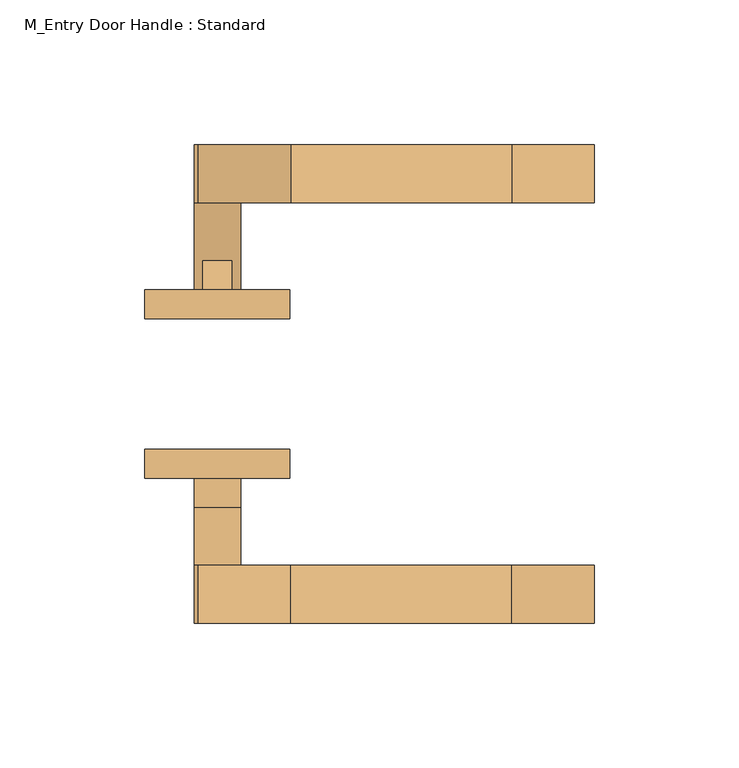
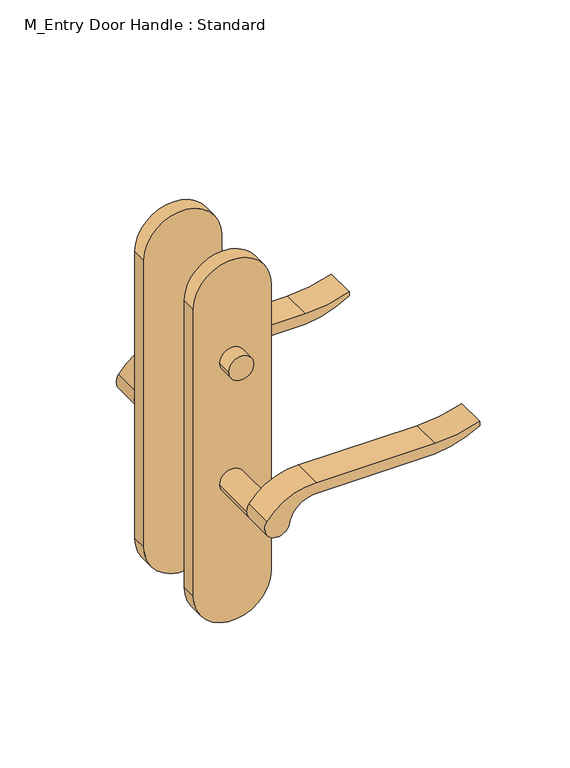
"""IFC4 building model written with IfcOpenShell, lengths in millimetres: door geometry, M_Entry Door Handle : Standard."""

from ifc_helpers import new_model, si_unit, point, frame, frame_2d, origin, origin_2d, place, context, project, spatial, polyline, circle_curve, trimmed, segment, composite_curve, outline, extrude, source, transform, mapped, element, save


def m_entry_door_handle_standard_7ac350b3(model_context):
    return source(origin(), model_context, "Body", "SweptSolid", [
        extrude(outline(polyline([(-5.0, 42.5), (5.0, 42.5), (5.0, 32.5), (-5.0, 32.5), (-5.0, 42.5)])), frame((0.0, 0.0, 67.5), z_axis=(0.0, 0.0, 1.0), x_axis=(1.0, 0.0, 0.0)), (0.0, 0.0, 1.0), 30.0),
        extrude(outline(composite_curve([segment(trimmed(circle_curve(frame_2d((82.5, 0.0)), 8.0), [point((82.5, 8.0))], [point((82.5, -8.0))], False, "CARTESIAN"), True, "CONTINUOUS"), segment(trimmed(circle_curve(frame_2d((82.5, 0.0)), 8.0), [point((82.5, -8.0))], [point((82.5, 8.0))], False, "CARTESIAN"), True, "CONTINUOUS")], self_intersect=False)), frame((0.0, -42.5, 0.0), z_axis=(0.0, 1.0, 0.0), x_axis=(0.0, 0.0, 1.0)), (0.0, 0.0, 1.0), 10.0),
        extrude(outline(composite_curve([segment(trimmed(circle_curve(origin_2d(), 8.0), [point((4.6523287, -6.5081363))], [point((0.0, 8.0))], False, "CARTESIAN"), True, "CONTINUOUS"), segment(trimmed(circle_curve(frame_2d((-5.1261387, 25.3861901)), 18.1261387), [point((0.0, 8.0))], [point((13.0, 25.3861901))], True, "CARTESIAN"), True, "CONTINUOUS"), segment(polyline([(13.0, 25.3861901), (13.0, 101.6435909)]), True, "CONTINUOUS"), segment(trimmed(circle_curve(frame_2d((72.2709207, 98.0603388)), 59.3791355), [point((13.0, 101.6435909))], [point((22.2135558, 130.0))], False, "CARTESIAN"), True, "CONTINUOUS"), segment(polyline([(22.2135558, 130.0), (25.0, 130.0)]), True, "CONTINUOUS"), segment(trimmed(circle_curve(frame_2d((103.2850638, 101.5772091)), 83.2850902), [point((25.0, 130.0))], [point((20.0, 101.6435909))], True, "CARTESIAN"), True, "CONTINUOUS"), segment(polyline([(20.0, 101.6435909), (20.0, 25.3674333)]), True, "CONTINUOUS"), segment(trimmed(circle_curve(frame_2d((-17.2444479, 23.6675129)), 37.2832219), [point((20.0, 25.3674333))], [point((4.6523287, -6.5081363))], False, "CARTESIAN"), True, "CONTINUOUS")], self_intersect=False)), frame((0.0, 62.5, 0.0), z_axis=(0.0, 1.0, 0.0), x_axis=(0.0, 0.0, 1.0)), (0.0, 0.0, 1.0), 20.0),
        extrude(outline(composite_curve([segment(trimmed(circle_curve(frame_2d((-5.1261318, 25.3861878)), 18.1261318), [point((-9.7e-06, 8.0))], [point((13.0, 25.3861878))], True, "CARTESIAN"), True, "CONTINUOUS"), segment(polyline([(13.0, 25.3861878), (13.0, 101.6435909)]), True, "CONTINUOUS"), segment(trimmed(circle_curve(frame_2d((72.2709207, 98.0603388)), 59.3791355), [point((13.0, 101.6435909))], [point((22.2135558, 130.0))], False, "CARTESIAN"), True, "CONTINUOUS"), segment(polyline([(22.2135558, 130.0), (25.0, 130.0)]), True, "CONTINUOUS"), segment(trimmed(circle_curve(frame_2d((103.2850638, 101.5772091)), 83.2850902), [point((25.0, 130.0))], [point((20.0, 101.6435909))], True, "CARTESIAN"), True, "CONTINUOUS"), segment(polyline([(20.0, 101.6435909), (20.0, 25.3674333)]), True, "CONTINUOUS"), segment(trimmed(circle_curve(frame_2d((-17.2444479, 23.6675129)), 37.2832219), [point((20.0, 25.3674333))], [point((4.6523287, -6.5081363))], False, "CARTESIAN"), True, "CONTINUOUS"), segment(trimmed(circle_curve(origin_2d(), 8.0), [point((4.6523287, -6.5081363))], [point((-9.7e-06, 8.0))], False, "CARTESIAN"), True, "CONTINUOUS")], self_intersect=False)), frame((0.0, -82.5, 0.0), z_axis=(0.0, 1.0, 0.0), x_axis=(0.0, 0.0, 1.0)), (0.0, 0.0, 1.0), 20.0),
        extrude(outline(composite_curve([segment(trimmed(circle_curve(origin_2d(), 8.0), [point((0.0, 8.0))], [point((0.0, -8.0))], False, "CARTESIAN"), True, "CONTINUOUS"), segment(trimmed(circle_curve(origin_2d(), 8.0), [point((0.0, -8.0))], [point((0.0, 8.0))], False, "CARTESIAN"), True, "CONTINUOUS")], self_intersect=False)), frame((0.0, 32.5, 0.0), z_axis=(0.0, 1.0, 0.0), x_axis=(0.0, 0.0, 1.0)), (0.0, 0.0, 1.0), 30.0),
        extrude(outline(composite_curve([segment(trimmed(circle_curve(origin_2d(), 8.0), [point((0.0, 8.0))], [point((0.0, -8.0))], False, "CARTESIAN"), True, "CONTINUOUS"), segment(trimmed(circle_curve(origin_2d(), 8.0), [point((0.0, -8.0))], [point((0.0, 8.0))], False, "CARTESIAN"), True, "CONTINUOUS")], self_intersect=False)), frame((0.0, -62.5, 0.0), z_axis=(0.0, 1.0, 0.0), x_axis=(0.0, 0.0, 1.0)), (0.0, 0.0, 1.0), 30.0),
        extrude(outline(composite_curve([segment(trimmed(circle_curve(frame_2d((-70.0, 0.0)), 25.0), [point((-70.0, -25.0))], [point((-70.0, 25.0))], False, "CARTESIAN"), True, "CONTINUOUS"), segment(polyline([(-70.0, 25.0), (125.0, 25.0)]), True, "CONTINUOUS"), segment(trimmed(circle_curve(frame_2d((125.0, 0.0)), 25.0), [point((125.0, 25.0))], [point((125.0, -25.0))], False, "CARTESIAN"), True, "CONTINUOUS"), segment(polyline([(125.0, -25.0), (-70.0, -25.0)]), True, "CONTINUOUS")], self_intersect=False)), frame((0.0, 22.5, 0.0), z_axis=(0.0, 1.0, 0.0), x_axis=(0.0, 0.0, 1.0)), (0.0, 0.0, 1.0), 10.0),
        extrude(outline(composite_curve([segment(trimmed(circle_curve(frame_2d((-70.0, 0.0)), 25.0), [point((-70.0, -25.0))], [point((-70.0, 25.0))], False, "CARTESIAN"), True, "CONTINUOUS"), segment(polyline([(-70.0, 25.0), (125.0, 25.0)]), True, "CONTINUOUS"), segment(trimmed(circle_curve(frame_2d((125.0, 0.0)), 25.0), [point((125.0, 25.0))], [point((125.0, -25.0))], False, "CARTESIAN"), True, "CONTINUOUS"), segment(polyline([(125.0, -25.0), (-70.0, -25.0)]), True, "CONTINUOUS")], self_intersect=False)), frame((0.0, -32.5, 0.0), z_axis=(0.0, 1.0, 0.0), x_axis=(0.0, 0.0, 1.0)), (0.0, 0.0, 1.0), 10.0),
    ])


if __name__ == "__main__":
    model = new_model("IFC4")
    model_context = context("Model", 3, world=origin())
    ifc_project = project(units=[si_unit("LENGTHUNIT", "METRE", prefix="MILLI")], contexts=[model_context])
    site = spatial("IfcSite", under=ifc_project)
    building = spatial("IfcBuilding", under=site)
    placement = place(None, origin())
    m_entry_door_handle_standard_shape = m_entry_door_handle_standard_7ac350b3(model_context)
    element("IfcDoor", 1, ObjectType="M_Entry Door Handle : Standard", at=placement, inside=building, context=model_context, shape_type="MappedRepresentation", body=[
        mapped(m_entry_door_handle_standard_shape, transform((0.0, 0.0, 0.0), x_axis=(1.0, 0.0, 0.0), y_axis=(0.0, 1.0, 0.0), z_axis=(0.0, 0.0, 1.0))),
    ])
    save(model, "model.ifc")

# Revit data of these elements
# Type "M_Entry Door Handle : Standard"
#   Type Mark = "50"
#   Analytic Construction = "<None>"
#   Thickness = 4.5 cm
#   Handle Material = Aluminum
#   Function = (empty or 0)
#   Construction Type = (empty or 0)
# Element 1 (IfcDoor, "M_Entry Door Handle : Standard")
#   Materials on its faces: "Aluminum"
# Materials
#   "Aluminum": class "Metal", colour RGB 247 247 247, transparency 0, Description = "Aluminum 6061", Cost = 0
